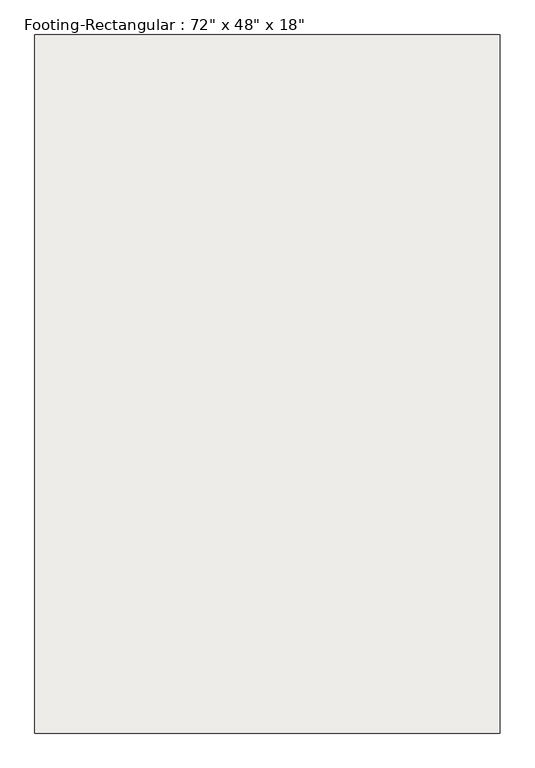
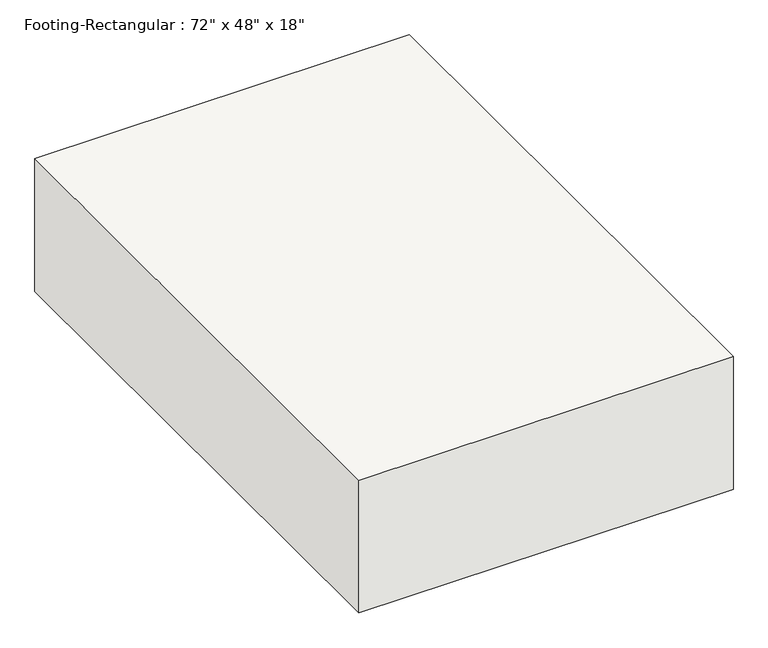
"""IFC4 building model written with IfcOpenShell, lengths in millimetres: slab geometry."""

import ifcopenshell
import ifcopenshell.guid

model = None  # the IFC model being written
_history = None  # IfcOwnerHistory: only IFC2X3 demands one
_inside = {}  # id of a spatial element -> (the spatial element, [elements in it])
_under = {}  # id of a project, library or spatial element -> (it, [spatial elements below it])
_declared = {}  # id of a project -> (the project, [libraries it declares])
_typed = {}  # id of a type object -> (the type object, [elements of that type])
_made_of = {}  # id of a material, layer set ... -> (it, [elements and type objects made of it])


def new_model(schema):
    """Start an empty IFC model of exactly this schema.

    Asked for "IFC4X3", IfcOpenShell would pick the latest addendum, in which some entities
    have other attributes; the version numbers below select the first issue.
    IFC2X3 requires an IfcOwnerHistory on every rooted entity: one is made here for all.
    """
    global model, _history
    if schema == "IFC4X3":
        model = ifcopenshell.file(schema_version=(4, 3, 0, 0))
    else:
        model = ifcopenshell.file(schema=schema)
    _inside.clear()
    _under.clear()
    _declared.clear()
    _typed.clear()
    _made_of.clear()
    _history = None
    if model.schema == "IFC2X3":
        org = make("IfcOrganization", Name="unknown")
        user = make(
            "IfcPersonAndOrganization",
            ThePerson=make("IfcPerson", FamilyName="unknown"),
            TheOrganization=org,
        )
        app = make(
            "IfcApplication",
            ApplicationDeveloper=org,
            Version="unknown",
            ApplicationFullName="unknown",
            ApplicationIdentifier="unknown",
        )
        _history = make(
            "IfcOwnerHistory",
            OwningUser=user,
            OwningApplication=app,
            ChangeAction="ADDED",
            CreationDate=0,
        )
    return model


def make(cls, **values):
    """One entity of the class cls with the attributes given. An attribute that is None is left unset."""
    return model.create_entity(
        cls, **{name: value for name, value in values.items() if value is not None}
    )


def rooted(cls, **values):
    """An entity with a GlobalId (a new one), such as an element, a storey or a relation."""
    return make(cls, GlobalId=ifcopenshell.guid.new(), OwnerHistory=_history, **values)


def si_unit(unit_type, name, prefix=None):
    """IfcSIUnit, for example si_unit("LENGTHUNIT", "METRE", prefix="MILLI")."""
    return make("IfcSIUnit", UnitType=unit_type, Prefix=prefix, Name=name)


def assignment(units):
    """IfcUnitAssignment: the units of a project."""
    return None if units is None else make("IfcUnitAssignment", Units=units)


def point(xyz):
    """IfcCartesianPoint."""
    return None if xyz is None else make("IfcCartesianPoint", Coordinates=xyz)


def direction(xyz):
    """IfcDirection."""
    return None if xyz is None else make("IfcDirection", DirectionRatios=xyz)


def frame(location, z_axis=None, x_axis=None):
    """IfcAxis2Placement3D, a coordinate frame: its origin and axes. An axis left out is left unset."""
    return make(
        "IfcAxis2Placement3D",
        Location=point(location),
        Axis=direction(z_axis),
        RefDirection=direction(x_axis),
    )


def origin():
    """The frame at (0, 0, 0) with its axes left unset."""
    return frame((0.0, 0.0, 0.0))


def place(relative_to, where):
    """IfcLocalPlacement: puts the frame where relative to a parent placement (None: the world)."""
    return make(
        "IfcLocalPlacement", PlacementRelTo=relative_to, RelativePlacement=where
    )


def context(
    kind, dimensions, precision=None, world=None, true_north=None, identifier=None
):
    """IfcGeometricRepresentationContext, for example the 3D "Model" context."""
    return make(
        "IfcGeometricRepresentationContext",
        ContextIdentifier=identifier,
        ContextType=kind,
        CoordinateSpaceDimension=dimensions,
        Precision=precision,
        WorldCoordinateSystem=world,
        TrueNorth=true_north,
    )


def project(units=None, contexts=None):
    """IfcProject with its units and contexts."""
    return rooted(
        "IfcProject",
        Name="project",
        RepresentationContexts=contexts,
        UnitsInContext=assignment(units),
    )


def spatial(cls, under=None, at=None, **own):
    """A site, building, storey or space (cls), placed at a placement, below another one or the project."""
    s = rooted(cls, ObjectPlacement=at, **own)
    if under is not None:
        _under.setdefault(under.id(), (under, []))[1].append(s)
    return s


def polyline(points):
    """IfcPolyline through the points."""
    return make("IfcPolyline", Points=[point(p) for p in points])


def outline(outer, holes=None, kind="AREA"):
    """IfcArbitraryClosedProfileDef: a profile drawn as a closed curve; with holes, ...WithVoids."""
    if holes is None:
        return make("IfcArbitraryClosedProfileDef", ProfileType=kind, OuterCurve=outer)
    return make(
        "IfcArbitraryProfileDefWithVoids",
        ProfileType=kind,
        OuterCurve=outer,
        InnerCurves=holes,
    )


def extrude(swept, where, along, depth):
    """IfcExtrudedAreaSolid: the profile swept, set in the frame where, extruded along a direction by depth."""
    return make(
        "IfcExtrudedAreaSolid",
        SweptArea=swept,
        Position=where,
        ExtrudedDirection=direction(along),
        Depth=depth,
    )


def shape(context_of_items, identifier, shape_type, items):
    """IfcShapeRepresentation: the items that make up one representation, for example the "Body"."""
    return make(
        "IfcShapeRepresentation",
        ContextOfItems=context_of_items,
        RepresentationIdentifier=identifier,
        RepresentationType=shape_type,
        Items=items,
    )


def source(mapping_origin, context_of_items, identifier, shape_type, items):
    """IfcRepresentationMap: a shape defined once, which mapped items show again and again."""
    return make(
        "IfcRepresentationMap",
        MappingOrigin=mapping_origin,
        MappedRepresentation=shape(context_of_items, identifier, shape_type, items),
    )


def transform(
    local_origin,
    x_axis=None,
    y_axis=None,
    z_axis=None,
    scale=None,
    scale2=None,
    scale3=None,
    uniform=True,
):
    """IfcCartesianTransformationOperator3D, or its non-uniform kind. x_axis, y_axis, z_axis: its Axis1, 2, 3."""
    if uniform:
        return make(
            "IfcCartesianTransformationOperator3D",
            Axis1=direction(x_axis),
            Axis2=direction(y_axis),
            LocalOrigin=point(local_origin),
            Scale=scale,
            Axis3=direction(z_axis),
        )
    return make(
        "IfcCartesianTransformationOperator3DnonUniform",
        Axis1=direction(x_axis),
        Axis2=direction(y_axis),
        LocalOrigin=point(local_origin),
        Scale=scale,
        Axis3=direction(z_axis),
        Scale2=scale2,
        Scale3=scale3,
    )


def mapped(mapping_source, mapping_target):
    """IfcMappedItem: shows the shape of a source again, moved by a transform."""
    return make(
        "IfcMappedItem", MappingSource=mapping_source, MappingTarget=mapping_target
    )


def made_of(thing, what):
    """Note that an element or type object is made of a material, layer set ...; save() writes the relation."""
    if what is not None:
        _made_of.setdefault(what.id(), (what, []))[1].append(thing)
    return thing


def element(
    cls,
    number,
    at=None,
    inside=None,
    cuts=None,
    type_object=None,
    material=None,
    context=None,
    identifier="Body",
    shape_type=None,
    held_by="IfcProductDefinitionShape",
    body=None,
    shapes=None,
    **own,
):
    """One element of the class cls, such as IfcWall. Its Tag is "e" and its number.

    at: its placement. inside: the storey or other place that contains it. cuts: it is an
    opening in that element (IfcRelVoidsElement). A single representation is given by context,
    identifier, shape_type and body (its items); several are given by shapes. held_by: the class
    of the entity that holds the representations. save() writes the other relations.
    """
    e = rooted(cls, Tag="e%d" % number, ObjectPlacement=at, **own)
    if body is not None:
        shapes = [shape(context, identifier, shape_type, body)]
    if shapes is not None:
        e.Representation = make(held_by, Representations=shapes)
    if inside is not None:
        _inside.setdefault(inside.id(), (inside, []))[1].append(e)
    if cuts is not None:
        rooted(
            "IfcRelVoidsElement", RelatingBuildingElement=cuts, RelatedOpeningElement=e
        )
    if type_object is not None:
        _typed.setdefault(type_object.id(), (type_object, []))[1].append(e)
    return made_of(e, material)


def aggregate(whole, parts):
    """IfcRelAggregates: a whole, such as a stair, and the parts it consists of."""
    return rooted("IfcRelAggregates", RelatingObject=whole, RelatedObjects=parts)


def save(model, path):
    """Write the relations noted so far, then the file.

    IfcRelAggregates (storeys below a building ...), IfcRelContainedInSpatialStructure (elements
    in a storey), IfcRelDefinesByType, IfcRelAssociatesMaterial and IfcRelDeclares: one each for
    every whole, place, type object, material and project.
    """
    for whole, parts in _under.values():
        aggregate(whole, parts)
    for where, things in _inside.values():
        rooted(
            "IfcRelContainedInSpatialStructure",
            RelatedElements=things,
            RelatingStructure=where,
        )
    for kind, things in _typed.values():
        rooted("IfcRelDefinesByType", RelatedObjects=things, RelatingType=kind)
    for what, things in _made_of.values():
        rooted("IfcRelAssociatesMaterial", RelatedObjects=things, RelatingMaterial=what)
    for by, libraries in _declared.values():
        rooted("IfcRelDeclares", RelatingContext=by, RelatedDefinitions=libraries)
    model.write(path)


def slab_5ba74754(model_context):
    return source(origin(), model_context, "Body", "SweptSolid", [
        extrude(outline(polyline([(609.6, 914.4), (609.6, -914.4), (-609.6, -914.4), (-609.6, 914.4), (609.6, 914.4)])), frame((0.0, 0.0, -457.2), z_axis=(0.0, 0.0, 1.0), x_axis=(1.0, 0.0, 0.0)), (0.0, 0.0, 1.0), 457.2),
    ])


if __name__ == "__main__":
    model = new_model("IFC4")
    model_context = context("Model", 3, world=origin())
    ifc_project = project(units=[si_unit("LENGTHUNIT", "METRE", prefix="MILLI")], contexts=[model_context])
    site = spatial("IfcSite", under=ifc_project)
    building = spatial("IfcBuilding", under=site)
    placement = place(None, origin())
    slab_shape = slab_5ba74754(model_context)
    element("IfcSlab", 1, ObjectType="Footing-Rectangular : 72\" x 48\" x 18\"", at=placement, inside=building, context=model_context, shape_type="MappedRepresentation", body=[
        mapped(slab_shape, transform((0.0, 0.0, 0.0), x_axis=(1.0, 0.0, 0.0), y_axis=(0.0, 1.0, 0.0), z_axis=(0.0, 0.0, 1.0))),
    ])
    save(model, "model.ifc")

# Revit data of these elements
# Project information
#   Project Issue Date = "Issue Date"
#   Project Status = "Project Status"
#   Client Name = "Owner"
#   Project Address = "Enter address here"
#   Project Name = "Project Name"
#   Project Number = "Project Number"
# Type "Footing-Rectangular : 72\" x 48\" x 18\""
#   Assembly Code = "A1010100"
#   Width = 4' - 0"
#   Length = 6' - 0"
#   Foundation Thickness = 1' - 6"
#   Structural Material [instance default] = Concrete, Cast-in-Place gray
# Element 1 (IfcSlab, "Footing-Rectangular : 72\" x 48\" x 18\"")
#   Materials on its faces: "Concrete, Cast-in-Place gray"
# Materials
#   "Concrete, Cast-in-Place gray": class "Concrete", colour RGB 192 192 192, transparency 0, Description = "Cast-in-place concrete", Cost = 0
